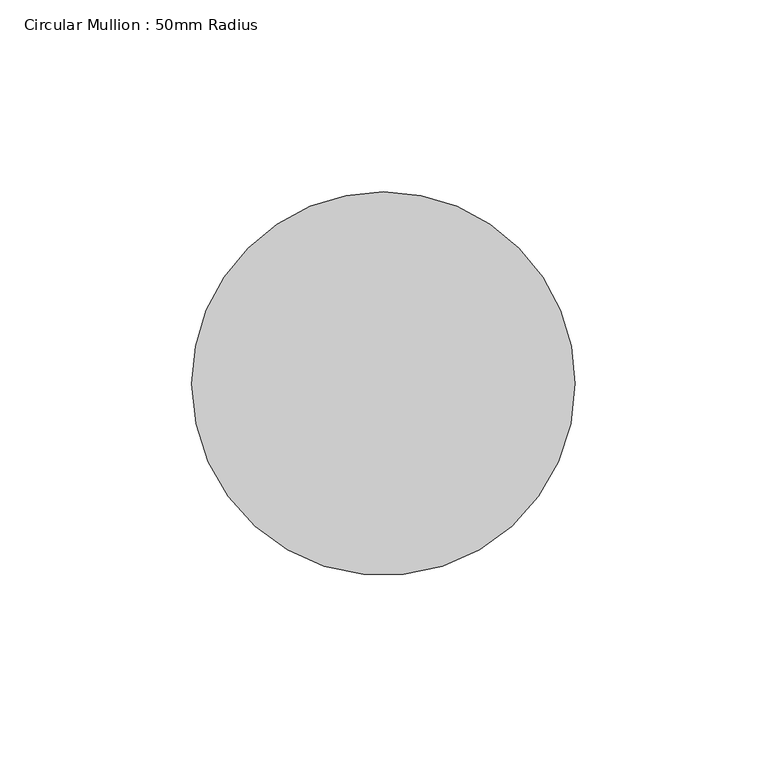
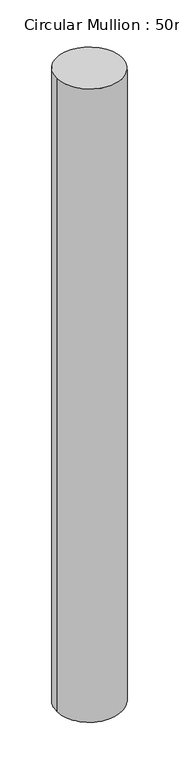
"""IFC4 building model written with IfcOpenShell, lengths in millimetres: member geometry, Circular Mullion : 50mm Radius."""

from ifc_helpers import new_model, si_unit, frame, origin, place, context, project, spatial, ellipse_curve, source, transform, mapped, element, save
from ifc_brep_helpers import plane_surface, cylinder_surface, advanced_brep


def circular_mullion_50mm_radius_d9435be7(model_context):
    return source(origin(), model_context, "Body", "AdvancedBrep", [
        advanced_brep(
        [(-100.0, 0.0, 1.5668085), (0.0, 0.0, 0.0), (0.0, 0.0, -1019.122961), (-100.0, 0.0, -1020.7129244)],
        [
            (0, 1, ellipse_curve(frame((-50.0, 0.0, 0.7834042), z_axis=(-0.01566440874184564, -0.014960931033782958, -0.999765370895277), x_axis=(-0.7229889061068856, -0.6905199768925874, 0.021661097816809534)), 50.0117342, 50.0)),
            (1, 2),
            (2, 3, ellipse_curve(frame((-50.0, 0.0, -1019.9179427), z_axis=(-0.015895793105750494, -0.0151819240867426, 0.9997583872829294), x_axis=(0.7229838558477079, 0.6905151534370156, 0.021981061335517815)), 50.0120836, 50.0)),
            (3, 0),
            (1, 0, ellipse_curve(frame((-50.0, 0.0, 0.7834042), z_axis=(-0.01566440874184564, -0.014960931033782958, -0.999765370895277), x_axis=(-0.7229889061068856, -0.6905199768925874, 0.021661097816809534)), 50.0117342, 50.0)),
            (3, 2, ellipse_curve(frame((-50.0, 0.0, -1019.9179427), z_axis=(-0.015895793105750494, -0.0151819240867426, 0.9997583872829294), x_axis=(0.7229838558477079, 0.6905151534370156, 0.021981061335517815)), 50.0120836, 50.0)),
        ],
        [
            cylinder_surface(frame((-50.0, 0.0, 0.0), z_axis=(0.0, 0.0, 1.0), x_axis=(1.0, 0.0, 0.0)), 50.0),
            plane_surface(frame((-210.519883, 220.4187352, 0.0), z_axis=(0.015664408741845645, 0.014960931033782961, 0.9997653708952772), x_axis=(0.7229889061068856, 0.6905199768925877, -0.0216610978168056))),
            plane_surface(frame((-210.519883, 220.4187352, -1019.122961), z_axis=(0.015895793105750494, 0.0151819240867426, -0.9997583872829294), x_axis=(0.7229838558477077, 0.6905151534370153, 0.02198106133553246))),
        ],
        [
            (0, [[1, 2, 3, 4]]),
            (0, [[5, -4, 6, -2]]),
            (1, [[-1, -5]]),
            (2, [[-6, -3]]),
        ],
    ),
    ])


if __name__ == "__main__":
    model = new_model("IFC4")
    model_context = context("Model", 3, world=origin())
    ifc_project = project(units=[si_unit("LENGTHUNIT", "METRE", prefix="MILLI")], contexts=[model_context])
    site = spatial("IfcSite", under=ifc_project)
    building = spatial("IfcBuilding", under=site)
    placement = place(None, origin())
    circular_mullion_50mm_radius_shape = circular_mullion_50mm_radius_d9435be7(model_context)
    element("IfcMember", 1, ObjectType="Circular Mullion : 50mm Radius", at=placement, inside=building, context=model_context, shape_type="MappedRepresentation", body=[
        mapped(circular_mullion_50mm_radius_shape, transform((0.0, 0.0, 0.0), x_axis=(1.0, 0.0, 0.0), y_axis=(0.0, 1.0, 0.0), z_axis=(0.0, 0.0, 1.0))),
    ])
    save(model, "model.ifc")

# Revit data of these elements
# Type "Circular Mullion : 50mm Radius"
#   built-in parameter 1007350 = 0.164042 (stored number, unit not read)
# Element 1 (IfcMember, "Circular Mullion : 50mm Radius")
#   Materials on its faces: "Aluminium"
# Materials
#   "Aluminium": class "Metal", colour RGB 247 247 247, transparency 0, Description = "Aluminium 6061", Cost = 0
